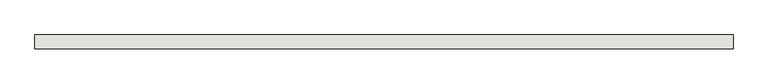
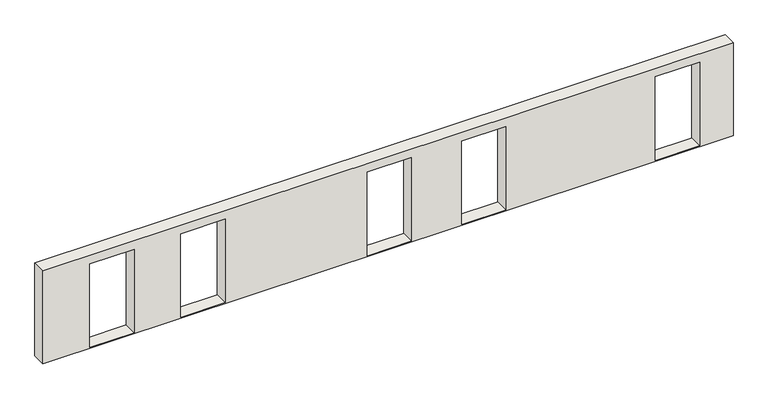
"""IFC4 building model written with IfcOpenShell, lengths in millimetres: wall geometry, 0_3d_modell."""

from ifc_helpers import new_model, si_unit, frame, origin, place, context, project, spatial, polyline, outline, extrude, source, transform, mapped, element, save


def wall_304ef8ab(model_context):
    return source(origin(), model_context, "Body", "SweptSolid", [
        extrude(outline(polyline([(0.0, 0.0), (0.0, 17652.8619019), (2510.0, 17652.8619019), (2510.0, 0.0), (0.0, 0.0)]), holes=[polyline([(20.0, 1200.0), (2280.0, 1200.0), (2280.0, 2335.0), (20.0, 2335.0), (20.0, 1200.0)]), polyline([(20.0, 3533.0664986), (2280.0, 3533.0664986), (2280.0, 4668.0664986), (20.0, 4668.0664986), (20.0, 3533.0664986)]), polyline([(20.0, 15668.259317), (2280.0, 15668.259317), (2280.0, 16803.259317), (20.0, 16803.259317), (20.0, 15668.259317)]), polyline([(20.0, 8292.897415), (2280.0, 8292.897415), (2280.0, 9427.897415), (20.0, 9427.897415), (20.0, 8292.897415)]), polyline([(20.0, 10707.5), (2280.0, 10707.5), (2280.0, 11842.5), (20.0, 11842.5), (20.0, 10707.5)])]), frame((0.0, 0.0, 0.0), z_axis=(0.0, 1.0, 0.0), x_axis=(0.0, 0.0, 1.0)), (0.0, 0.0, 1.0), 350.0),
    ])


if __name__ == "__main__":
    model = new_model("IFC4")
    model_context = context("Model", 3, world=origin())
    ifc_project = project(units=[si_unit("LENGTHUNIT", "METRE", prefix="MILLI")], contexts=[model_context])
    site = spatial("IfcSite", under=ifc_project)
    building = spatial("IfcBuilding", under=site)
    placement = place(None, origin())
    wall_shape = wall_304ef8ab(model_context)
    element("IfcWall", 1, ObjectType="0_3d_modell", at=placement, inside=building, context=model_context, shape_type="MappedRepresentation", body=[
        mapped(wall_shape, transform((0.0, 0.0, 0.0), x_axis=(1.0, 0.0, 0.0), y_axis=(0.0, 1.0, 0.0), z_axis=(0.0, 0.0, 1.0))),
    ])
    save(model, "model.ifc")

# Revit data of these elements
# Element 1 (IfcWall, "0_3d_modell")
#   Materials on its faces: "holzschalung"
# Materials
#   "holzschalung": class "Unassigned", colour RGB 128 128 128, transparency 0
